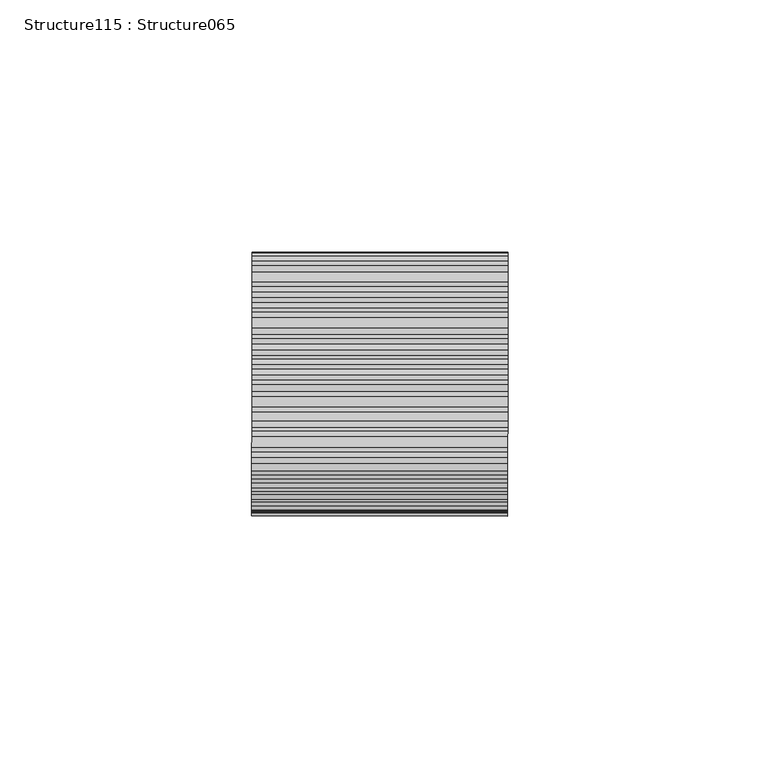
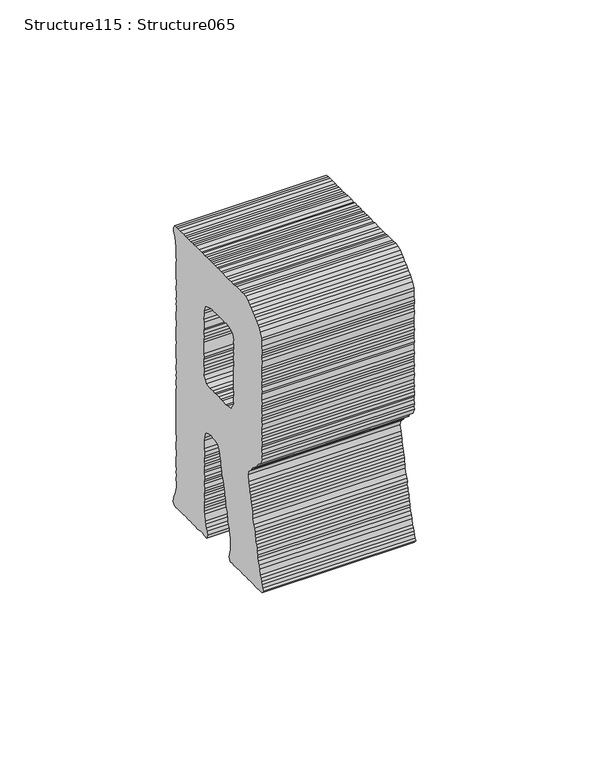
"""IFC4 building model written with IfcOpenShell, lengths in millimetres: proxy geometry, Structure115 : Structure065."""

from ifc_helpers import new_model, si_unit, frame, origin, place, context, project, spatial, polyline, outline, extrude, source, transform, mapped, element, save


def structure115_structure065_5d93ba90(model_context):
    return source(origin(), model_context, "Body", "SweptSolid", [
        extrude(outline(polyline([(0.7871188, 0.0), (1.9467099, -0.1934423), (2.8611126, -0.2132328), (4.1212942, -0.5562053), (5.0176609, -0.7057366), (5.8930671, -0.9830781), (7.2176513, -0.9399881), (7.9671776, -1.1977733), (10.1456225, -1.5611803), (11.3169321, -1.6238278), (12.3202067, -1.9239432), (13.220785, -2.0741771), (14.2235918, -2.3727715), (15.4221794, -2.3086628), (16.5332978, -2.7580754), (17.4474664, -2.7792697), (18.628954, -2.8436152), (20.3760226, -3.3991165), (21.6573988, -3.612875), (22.5973246, -3.5056165), (23.7042315, -3.9543264), (24.6497726, -3.8480047), (25.7998876, -4.0398662), (26.5259967, -4.4250517), (27.5508168, -4.5960116), (28.8750501, -4.5528631), (29.8605229, -4.9813155), (30.8000977, -4.8739985), (32.5717532, -6.0908565), (32.9377317, -7.0757454), (33.5964553, -7.8432491), (34.5198072, -8.6548979), (35.1339188, -9.6790159), (36.0291146, -11.4098043), (36.9291659, -12.3503158), (37.5875383, -13.1199252), (37.9967252, -13.8458014), (39.5794443, -14.6361388), (41.715559, -14.4661751), (43.0356389, -14.4241375), (43.9753304, -14.3182828), (45.1310609, -14.5110811), (46.0922399, -14.2742577), (47.0321656, -14.1669992), (48.2092074, -14.2320459), (49.1644782, -13.9960405), (50.1096681, -13.8918246), (51.1536356, -13.9328683), (52.2245298, -13.8492615), (53.5020455, -14.0623759), (55.3872199, -13.8483862), (56.4950633, -13.5065262), (57.6901412, -13.4418321), (58.8221031, -13.7641364), (59.6518448, -13.5086333), (60.8291209, -13.5722761), (61.6842107, -13.1864483), (62.8570992, -13.2526058), (63.8005346, -13.1459328), (64.9935066, -13.0808873), (65.8902243, -13.2304773), (66.9632246, -13.1450575), (68.1987025, -12.8252108), (69.3917916, -12.7594635), (71.3806564, -12.698046), (72.2372083, -12.3142657), (73.3027212, -12.2283183), (74.1379616, -11.9722896), (75.3345601, -11.909292), (76.060085, -11.5022109), (76.9541114, -12.4420781), (76.9148807, -13.4881518), (76.654873, -14.2358644), (76.6153496, -15.2836929), (76.4231953, -16.4355628), (76.1203305, -17.4401823), (75.7994879, -19.363475), (75.9089108, -20.303401), (75.4361395, -21.5415689), (75.3958554, -23.3789145), (75.0550475, -24.6369321), (74.5630694, -27.5860978), (74.5408215, -28.5044193), (74.1318675, -29.3600344), (74.2202717, -30.4259573), (72.7677599, -31.2380719), (71.9348595, -30.7059292), (70.9319944, -30.4055214), (69.81877, -29.9557576), (69.092661, -29.5705722), (67.0454774, -29.2290621), (65.8897469, -29.0362638), (64.9073151, -29.4004878), (63.9889933, -29.3804043), (62.8179181, -29.3141886), (61.8295198, -29.6774173), (60.6364307, -29.7431647), (59.5910013, -29.697909), (58.5414768, -29.6555776), (57.4974509, -29.6127205), (56.5096379, -29.9746039), (55.3383286, -29.909792), (54.2921965, -29.868748), (53.1997567, -30.0815102), (52.2660901, -30.1880092), (51.3634061, -30.0374239), (50.1703755, -30.1028203), (49.1034001, -30.1888844), (48.011253, -30.3998918), (47.2025297, -30.5315625), (45.9829235, -30.721668), (45.0646604, -30.6990691), (43.8681202, -30.76388), (42.9281945, -30.8711385), (41.6450635, -30.6570873), (40.8369841, -30.7848975), (39.744193, -30.9997654), (38.4199597, -31.0429139), (36.6021707, -31.6617044), (35.708143, -33.0918512), (35.4943845, -34.3732273), (35.1130014, -35.098167), (35.152289, -36.4239207), (35.3651098, -38.3031284), (36.0274012, -39.073031), (37.503973, -39.7125505), (38.6111139, -40.162021), (41.55677, -40.6534136), (42.628074, -40.5673501), (43.9094502, -40.7811085), (44.8909452, -41.2096189), (45.9402356, -41.2533541), (46.7273547, -41.2511898), (47.7284064, -41.5516557), (49.0153982, -41.766351), (49.8872947, -42.043107), (51.0842445, -41.9780036), (52.1143292, -42.1498418), (52.8581229, -42.4073921), (53.8647903, -42.7066306), (55.1894917, -42.6628386), (56.2136099, -42.8336815), (57.0677043, -43.2409389), (57.964422, -43.3905288), (59.1613718, -43.3254254), (60.2702675, -43.7751887), (61.3142934, -43.8180457), (62.0853652, -43.9466754), (63.2180294, -44.2669326), (64.1538606, -44.1582696), (66.5064238, -44.2866665), (67.3413129, -44.0327435), (68.6659557, -43.9893025), (69.5168336, -43.6049365), (70.7154797, -43.5404768), (71.9110832, -44.2684002), (71.5698656, -45.5288744), (71.1417648, -46.5100771), (70.9918236, -47.4089006), (70.9678209, -48.3269294), (70.9073373, -49.5004036), (70.6044725, -50.5050232), (70.5864362, -51.4240474), (70.415242, -52.4502714), (70.008687, -53.3023186), (69.96308, -54.3498537), (69.5997902, -56.5275967), (69.5604424, -57.5743723), (69.2792403, -58.4491345), (68.9155992, -60.6289833), (68.8979142, -61.5459016), (68.7482657, -62.4429702), (67.4443489, -63.1492881), (66.3524357, -62.5739371), (65.5024946, -62.1655689), (64.4335891, -61.46311), (63.7054328, -61.0772223), (61.7402195, -60.2227167), (60.7157502, -60.0518153), (58.6206793, -59.9649302), (57.7721999, -59.5607739), (56.4677577, -59.4723099), (55.5881396, -59.1964302), (54.5210475, -59.2810319), (51.5715307, -58.7889952), (50.5917902, -58.3629421), (49.5673209, -58.1920407), (48.2590182, -58.1029327), (46.3434468, -57.7833781), (45.336428, -57.4862455), (44.3137136, -57.3156369), (43.2682842, -57.2703813), (39.296404, -56.6077945), (38.2502721, -56.5667504), (37.243956, -56.2654062), (35.9388112, -56.1811538), (34.9164477, -56.0106037), (34.1666876, -55.7520581), (33.1226615, -55.7113653), (31.8353188, -55.4966116), (30.8325123, -55.1958529), (29.9414101, -55.0471997), (29.0174143, -55.0265303), (27.8672993, -54.8346688), (27.0093438, -54.4289318), (25.8361629, -54.3623647), (24.7921367, -54.3216719), (23.6846447, -53.8743073), (22.8887519, -53.8706793), (21.8852429, -53.5741322), (20.5829065, -53.4860194), (19.5371255, -53.4450339), (18.8100804, -53.0611353), (17.5269493, -52.8470841), (16.718519, -52.9748356), (15.5589279, -52.7813933), (14.6894885, -52.5028828), (13.6437075, -52.4618973), (12.3780276, -52.1172862), (11.6335313, -51.8639474), (10.4624561, -51.7977316), (8.2783958, -51.4333879), (7.487767, -51.4349668), (6.3589637, -51.1131894), (5.4835572, -50.8380123), (4.3271248, -50.6450969), (3.3881352, -50.7510686), (2.259332, -50.4292911), (1.3356871, -50.4086803), (0.1004434, -49.9400043), (-0.9278864, -49.7684589), (-1.97121, -49.7235545), (-2.7160573, -49.4701572), (-3.7667512, -49.4240234), (-4.7685054, -49.127769), (-6.0502326, -48.913952), (-6.8639273, -49.0408253), (-8.1236408, -48.6972095), (-8.8741036, -48.4428755), (-9.896116, -48.2723839), (-10.9635591, -48.3569271), (-11.9698753, -48.0555829), (-13.2512515, -47.8418244), (-14.0439861, -47.843052), (-16.0908187, -47.5016005), (-17.2039264, -47.0532992), (-18.2692637, -47.1381936), (-19.3977159, -46.8164747), (-20.4498143, -46.7744354), (-21.3248692, -46.4949881), (-23.5459373, -46.3892487), (-24.6132635, -46.4752543), (-25.468002, -46.8589763), (-26.5569911, -47.0748393), (-27.732161, -47.0093834), (-28.6765316, -46.3237312), (-28.6309247, -45.2761961), (-28.4816275, -44.3812333), (-28.1419891, -43.1194134), (-27.9467337, -41.1748095), (-27.6717907, -40.3008068), (-27.6265937, -39.2557284), (-27.4341467, -38.1021037), (-27.1585597, -37.2242404), (-27.0919341, -36.0507086), (-26.8380098, -35.3027026), (-26.7927543, -34.2572731), (-26.450366, -32.204825), (-26.1112545, -30.9461638), (-26.2363148, -30.1345751), (-25.7904705, -29.0232221), (-25.851655, -27.8287298), (-25.5527093, -26.8238171), (-25.2987265, -26.0754601), (-25.3808712, -25.0066136), (-25.1035297, -24.1312073), (-25.039127, -22.9580261), (-24.7405326, -21.9552192), (-24.7183429, -21.0350843), (-24.2514799, -19.7977346), (-24.205873, -18.7501993), (-23.7377804, -16.7183605), (-23.5672889, -15.696348), (-23.2893034, -14.0299623), (-23.0751936, -12.7464803), (-23.0728537, -11.9583088), (-23.0293526, -10.9104224), (-22.6659456, -8.7319775), (-22.3886627, -7.8569222), (-22.3451616, -6.8090358), (-21.89961, -5.6994375), (-21.1256712, -4.2496184), (-20.1054129, -3.6283696), (-19.3334628, -2.9646161), (-18.3028512, -2.3461766), (-17.4942452, -1.4302533), (-16.8743997, -0.871711), (-16.0026199, -0.3598857), (-15.0773951, 0.4096054), (-14.3584222, 0.8141722), (-13.2017553, 1.4119438), (-11.4074421, 1.902983), (-10.4894129, 1.8811446), (-8.4366139, 1.5386978), (-7.1375527, 1.4547388), (-6.3622692, 1.3254065), (-5.381008, 0.8976567), (-4.3582936, 0.7270481), (-3.2909673, 0.8130537), (-1.0241182, 0.1708428), (0.0, 0.0), (0.7871188, 0.0)]), holes=[polyline([(19.0863815, -31.6360536), (19.4317522, -30.3766329), (19.4281256, -29.5874661), (19.6422354, -28.3039841), (20.0937534, -27.1953812), (20.1372546, -26.1474947), (20.6074529, -24.1160071), (20.4976205, -23.1763735), (20.5710904, -21.2136178), (19.7325749, -20.6783741), (18.4726861, -19.546528), (17.5550665, -19.5243972), (16.2736902, -19.3106387), (15.5235202, -19.0545498), (14.3695447, -18.8620443), (13.4550837, -18.8404404), (12.4330713, -18.6699488), (11.1240659, -18.5850524), (9.0751274, -18.2432497), (8.0688113, -17.9419055), (7.1500799, -17.9221143), (6.2533623, -17.7725244), (5.1461629, -17.323405), (4.2494452, -17.173815), (3.0724619, -17.1084173), (2.1753932, -16.9587688), (1.1739318, -16.6607596), (-0.0030516, -16.5953619), (-0.8785164, -16.3183714), (-2.0342468, -16.1255731), (-2.9525684, -16.1033252), (-3.8224177, -15.8272714), (-5.4698908, -16.2122211), (-6.3692412, -16.8525575), (-7.4590496, -18.6454073), (-7.6303023, -19.6719823), (-7.501381, -20.4820507), (-7.9294821, -21.4654176), (-8.4641417, -24.6704375), (-8.5516107, -25.9710776), (-8.5489789, -26.7618821), (-8.9767287, -27.7431433), (-8.8910744, -28.8125754), (-8.550444, -30.714908), (-8.1628609, -31.5681261), (-6.711052, -32.3366251), (-5.8146853, -32.4861565), (-3.5476025, -33.1291279), (-2.6117712, -33.0204648), (-0.4336773, -33.3838132), (0.2930166, -33.7698177), (1.4700584, -33.8348644), (2.3884388, -33.854597), (3.6233312, -34.3253789), (4.4136088, -34.3259058), (8.3875947, -34.9888439), (9.5628822, -35.0514336), (10.4169766, -35.458691), (11.4467103, -35.6304706), (12.6184877, -35.694639), (13.5372191, -35.7144302), (14.5651979, -35.885917), (15.8210508, -36.2288888), (17.2098622, -35.8007894), (18.2192791, -35.3115639), (19.0465068, -33.4731068), (19.0863815, -31.6360536)])]), frame((-56111.2741132, 291797.4761843, -297.3854876), z_axis=(-0.9999998917542984, 0.0004652863545059616, 0.0), x_axis=(-7.65608205057226e-05, -0.16454557818285864, -0.9863694778524473)), (0.0, 0.0, 1.0), 50.8),
    ])


if __name__ == "__main__":
    model = new_model("IFC4")
    model_context = context("Model", 3, world=origin())
    ifc_project = project(units=[si_unit("LENGTHUNIT", "METRE", prefix="MILLI")], contexts=[model_context])
    site = spatial("IfcSite", under=ifc_project)
    building = spatial("IfcBuilding", under=site)
    placement = place(None, origin())
    structure115_structure065_shape = structure115_structure065_5d93ba90(model_context)
    element("IfcBuildingElementProxy", 1, Name="Structure115 : Structure065", ObjectType="Structure115 : Structure065", at=placement, inside=building, context=model_context, shape_type="MappedRepresentation", body=[
        mapped(structure115_structure065_shape, transform((0.0, 0.0, 0.0), x_axis=(1.0, 0.0, 0.0), y_axis=(0.0, 1.0, 0.0), z_axis=(0.0, 0.0, 1.0))),
    ])
    save(model, "model.ifc")

# Revit data of these elements
# Type "Structure115 : Structure065"
#   NameOverride = "Structure065"
# Element 1 (IfcBuildingElementProxy, "Structure115 : Structure065")
#   Materials on its faces: "BRUSHED ALUMINUM LETTERING"
# Materials
#   "BRUSHED ALUMINUM LETTERING": class "Unassigned", colour RGB 169 181 186, transparency 0, Cost = 0
